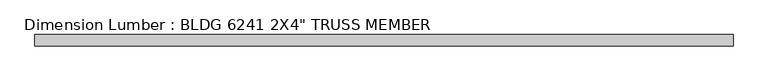
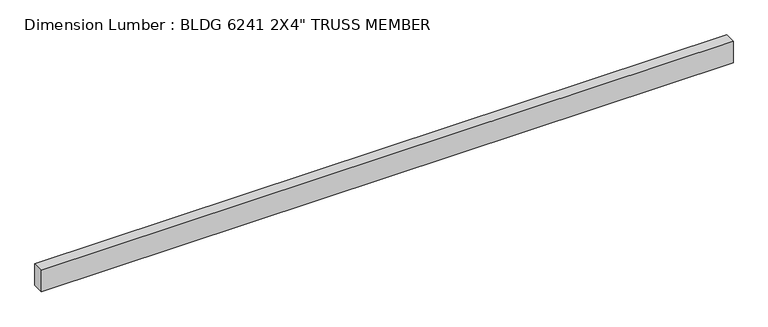
"""IFC4 building model written with IfcOpenShell, lengths in millimetres: beam geometry."""

import ifcopenshell
import ifcopenshell.guid

model = None  # the IFC model being written
_history = None  # IfcOwnerHistory: only IFC2X3 demands one
_inside = {}  # id of a spatial element -> (the spatial element, [elements in it])
_under = {}  # id of a project, library or spatial element -> (it, [spatial elements below it])
_declared = {}  # id of a project -> (the project, [libraries it declares])
_typed = {}  # id of a type object -> (the type object, [elements of that type])
_made_of = {}  # id of a material, layer set ... -> (it, [elements and type objects made of it])


def new_model(schema):
    """Start an empty IFC model of exactly this schema.

    Asked for "IFC4X3", IfcOpenShell would pick the latest addendum, in which some entities
    have other attributes; the version numbers below select the first issue.
    IFC2X3 requires an IfcOwnerHistory on every rooted entity: one is made here for all.
    """
    global model, _history
    if schema == "IFC4X3":
        model = ifcopenshell.file(schema_version=(4, 3, 0, 0))
    else:
        model = ifcopenshell.file(schema=schema)
    _inside.clear()
    _under.clear()
    _declared.clear()
    _typed.clear()
    _made_of.clear()
    _history = None
    if model.schema == "IFC2X3":
        org = make("IfcOrganization", Name="unknown")
        user = make(
            "IfcPersonAndOrganization",
            ThePerson=make("IfcPerson", FamilyName="unknown"),
            TheOrganization=org,
        )
        app = make(
            "IfcApplication",
            ApplicationDeveloper=org,
            Version="unknown",
            ApplicationFullName="unknown",
            ApplicationIdentifier="unknown",
        )
        _history = make(
            "IfcOwnerHistory",
            OwningUser=user,
            OwningApplication=app,
            ChangeAction="ADDED",
            CreationDate=0,
        )
    return model


def make(cls, **values):
    """One entity of the class cls with the attributes given. An attribute that is None is left unset."""
    return model.create_entity(
        cls, **{name: value for name, value in values.items() if value is not None}
    )


def rooted(cls, **values):
    """An entity with a GlobalId (a new one), such as an element, a storey or a relation."""
    return make(cls, GlobalId=ifcopenshell.guid.new(), OwnerHistory=_history, **values)


def si_unit(unit_type, name, prefix=None):
    """IfcSIUnit, for example si_unit("LENGTHUNIT", "METRE", prefix="MILLI")."""
    return make("IfcSIUnit", UnitType=unit_type, Prefix=prefix, Name=name)


def assignment(units):
    """IfcUnitAssignment: the units of a project."""
    return None if units is None else make("IfcUnitAssignment", Units=units)


def point(xyz):
    """IfcCartesianPoint."""
    return None if xyz is None else make("IfcCartesianPoint", Coordinates=xyz)


def direction(xyz):
    """IfcDirection."""
    return None if xyz is None else make("IfcDirection", DirectionRatios=xyz)


def frame(location, z_axis=None, x_axis=None):
    """IfcAxis2Placement3D, a coordinate frame: its origin and axes. An axis left out is left unset."""
    return make(
        "IfcAxis2Placement3D",
        Location=point(location),
        Axis=direction(z_axis),
        RefDirection=direction(x_axis),
    )


def origin():
    """The frame at (0, 0, 0) with its axes left unset."""
    return frame((0.0, 0.0, 0.0))


def place(relative_to, where):
    """IfcLocalPlacement: puts the frame where relative to a parent placement (None: the world)."""
    return make(
        "IfcLocalPlacement", PlacementRelTo=relative_to, RelativePlacement=where
    )


def context(
    kind, dimensions, precision=None, world=None, true_north=None, identifier=None
):
    """IfcGeometricRepresentationContext, for example the 3D "Model" context."""
    return make(
        "IfcGeometricRepresentationContext",
        ContextIdentifier=identifier,
        ContextType=kind,
        CoordinateSpaceDimension=dimensions,
        Precision=precision,
        WorldCoordinateSystem=world,
        TrueNorth=true_north,
    )


def project(units=None, contexts=None):
    """IfcProject with its units and contexts."""
    return rooted(
        "IfcProject",
        Name="project",
        RepresentationContexts=contexts,
        UnitsInContext=assignment(units),
    )


def spatial(cls, under=None, at=None, **own):
    """A site, building, storey or space (cls), placed at a placement, below another one or the project."""
    s = rooted(cls, ObjectPlacement=at, **own)
    if under is not None:
        _under.setdefault(under.id(), (under, []))[1].append(s)
    return s


def polyline(points):
    """IfcPolyline through the points."""
    return make("IfcPolyline", Points=[point(p) for p in points])


def outline(outer, holes=None, kind="AREA"):
    """IfcArbitraryClosedProfileDef: a profile drawn as a closed curve; with holes, ...WithVoids."""
    if holes is None:
        return make("IfcArbitraryClosedProfileDef", ProfileType=kind, OuterCurve=outer)
    return make(
        "IfcArbitraryProfileDefWithVoids",
        ProfileType=kind,
        OuterCurve=outer,
        InnerCurves=holes,
    )


def extrude(swept, where, along, depth):
    """IfcExtrudedAreaSolid: the profile swept, set in the frame where, extruded along a direction by depth."""
    return make(
        "IfcExtrudedAreaSolid",
        SweptArea=swept,
        Position=where,
        ExtrudedDirection=direction(along),
        Depth=depth,
    )


def shape(context_of_items, identifier, shape_type, items):
    """IfcShapeRepresentation: the items that make up one representation, for example the "Body"."""
    return make(
        "IfcShapeRepresentation",
        ContextOfItems=context_of_items,
        RepresentationIdentifier=identifier,
        RepresentationType=shape_type,
        Items=items,
    )


def source(mapping_origin, context_of_items, identifier, shape_type, items):
    """IfcRepresentationMap: a shape defined once, which mapped items show again and again."""
    return make(
        "IfcRepresentationMap",
        MappingOrigin=mapping_origin,
        MappedRepresentation=shape(context_of_items, identifier, shape_type, items),
    )


def transform(
    local_origin,
    x_axis=None,
    y_axis=None,
    z_axis=None,
    scale=None,
    scale2=None,
    scale3=None,
    uniform=True,
):
    """IfcCartesianTransformationOperator3D, or its non-uniform kind. x_axis, y_axis, z_axis: its Axis1, 2, 3."""
    if uniform:
        return make(
            "IfcCartesianTransformationOperator3D",
            Axis1=direction(x_axis),
            Axis2=direction(y_axis),
            LocalOrigin=point(local_origin),
            Scale=scale,
            Axis3=direction(z_axis),
        )
    return make(
        "IfcCartesianTransformationOperator3DnonUniform",
        Axis1=direction(x_axis),
        Axis2=direction(y_axis),
        LocalOrigin=point(local_origin),
        Scale=scale,
        Axis3=direction(z_axis),
        Scale2=scale2,
        Scale3=scale3,
    )


def mapped(mapping_source, mapping_target):
    """IfcMappedItem: shows the shape of a source again, moved by a transform."""
    return make(
        "IfcMappedItem", MappingSource=mapping_source, MappingTarget=mapping_target
    )


def made_of(thing, what):
    """Note that an element or type object is made of a material, layer set ...; save() writes the relation."""
    if what is not None:
        _made_of.setdefault(what.id(), (what, []))[1].append(thing)
    return thing


def element(
    cls,
    number,
    at=None,
    inside=None,
    cuts=None,
    type_object=None,
    material=None,
    context=None,
    identifier="Body",
    shape_type=None,
    held_by="IfcProductDefinitionShape",
    body=None,
    shapes=None,
    **own,
):
    """One element of the class cls, such as IfcWall. Its Tag is "e" and its number.

    at: its placement. inside: the storey or other place that contains it. cuts: it is an
    opening in that element (IfcRelVoidsElement). A single representation is given by context,
    identifier, shape_type and body (its items); several are given by shapes. held_by: the class
    of the entity that holds the representations. save() writes the other relations.
    """
    e = rooted(cls, Tag="e%d" % number, ObjectPlacement=at, **own)
    if body is not None:
        shapes = [shape(context, identifier, shape_type, body)]
    if shapes is not None:
        e.Representation = make(held_by, Representations=shapes)
    if inside is not None:
        _inside.setdefault(inside.id(), (inside, []))[1].append(e)
    if cuts is not None:
        rooted(
            "IfcRelVoidsElement", RelatingBuildingElement=cuts, RelatedOpeningElement=e
        )
    if type_object is not None:
        _typed.setdefault(type_object.id(), (type_object, []))[1].append(e)
    return made_of(e, material)


def aggregate(whole, parts):
    """IfcRelAggregates: a whole, such as a stair, and the parts it consists of."""
    return rooted("IfcRelAggregates", RelatingObject=whole, RelatedObjects=parts)


def save(model, path):
    """Write the relations noted so far, then the file.

    IfcRelAggregates (storeys below a building ...), IfcRelContainedInSpatialStructure (elements
    in a storey), IfcRelDefinesByType, IfcRelAssociatesMaterial and IfcRelDeclares: one each for
    every whole, place, type object, material and project.
    """
    for whole, parts in _under.values():
        aggregate(whole, parts)
    for where, things in _inside.values():
        rooted(
            "IfcRelContainedInSpatialStructure",
            RelatedElements=things,
            RelatingStructure=where,
        )
    for kind, things in _typed.values():
        rooted("IfcRelDefinesByType", RelatedObjects=things, RelatingType=kind)
    for what, things in _made_of.values():
        rooted("IfcRelAssociatesMaterial", RelatedObjects=things, RelatingMaterial=what)
    for by, libraries in _declared.values():
        rooted("IfcRelDeclares", RelatingContext=by, RelatedDefinitions=libraries)
    model.write(path)


def beam_fc8bf4ae(model_context):
    return source(origin(), model_context, "Body", "SweptSolid", [
        extrude(outline(polyline([(1562.6646551, 25.4), (1562.6646551, -25.4), (-1550.1468127, -25.4), (-1550.1468127, 25.4), (1562.6646551, 25.4)])), frame((0.0, 0.0, -50.8), z_axis=(0.0, 0.0, 1.0), x_axis=(1.0, 0.0, 0.0)), (0.0, 0.0, 1.0), 101.6),
    ])


if __name__ == "__main__":
    model = new_model("IFC4")
    model_context = context("Model", 3, world=origin())
    ifc_project = project(units=[si_unit("LENGTHUNIT", "METRE", prefix="MILLI")], contexts=[model_context])
    site = spatial("IfcSite", under=ifc_project)
    building = spatial("IfcBuilding", under=site)
    placement = place(None, origin())
    beam_shape = beam_fc8bf4ae(model_context)
    element("IfcBeam", 1, ObjectType="Dimension Lumber : BLDG 6241 2X4\" TRUSS MEMBER", at=placement, inside=building, context=model_context, shape_type="MappedRepresentation", body=[
        mapped(beam_shape, transform((0.0, 0.0, 0.0), x_axis=(1.0, 0.0, 0.0), y_axis=(0.0, 1.0, 0.0), z_axis=(0.0, 0.0, 1.0))),
    ])
    save(model, "model.ifc")

# Revit data of these elements
# Type "Dimension Lumber : BLDG 6241 2X4\" TRUSS MEMBER"
#   Assembly Code = "B10"
#   A = 0.273472 SF
#   Length [instance default] = 5' - 0"
#   b = 0' - 2"
#   d = 0' - 4"
#   Structural Material [instance default] = Softwood, Lumber
# Element 1 (IfcBeam, "Dimension Lumber : BLDG 6241 2X4\" TRUSS MEMBER")
#   Materials on its faces: "Softwood, Lumber"
# Materials
#   "Softwood, Lumber": class "Wood", colour RGB 223 192 134, transparency 0, Description = "Pinus Echinata", Cost = 0
